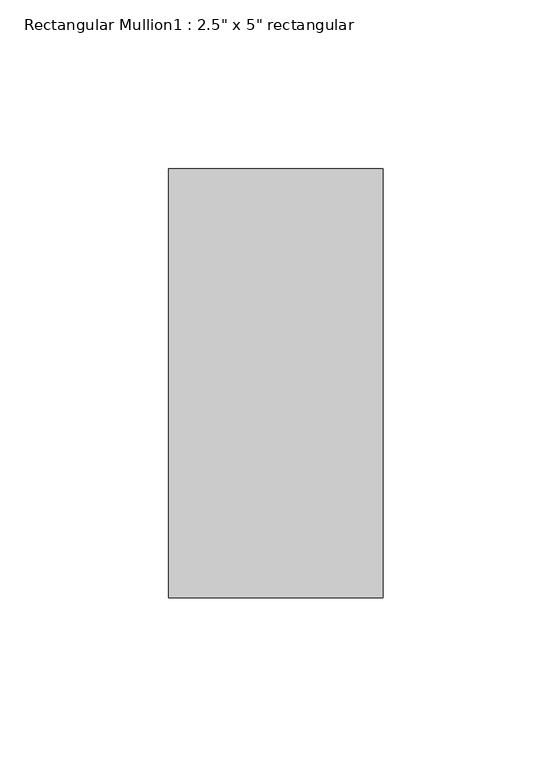
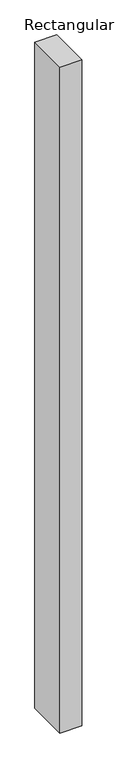
"""IFC4 building model written with IfcOpenShell, lengths in millimetres: member geometry."""

from ifc_helpers import new_model, si_unit, frame, origin, place, context, project, spatial, polyline, outline, extrude, source, transform, mapped, element, save


def member_08becc7e(model_context):
    return source(origin(), model_context, "Body", "SweptSolid", [
        extrude(outline(polyline([(0.0, 63.5), (0.0, -63.5), (-63.5, -63.5), (-63.5, 63.5), (0.0, 63.5)])), frame((0.0, 0.0, -2059.94), z_axis=(0.0, 0.0, 1.0), x_axis=(1.0, 0.0, 0.0)), (0.0, 0.0, 1.0), 2059.94),
    ])


if __name__ == "__main__":
    model = new_model("IFC4")
    model_context = context("Model", 3, world=origin())
    ifc_project = project(units=[si_unit("LENGTHUNIT", "METRE", prefix="MILLI")], contexts=[model_context])
    site = spatial("IfcSite", under=ifc_project)
    building = spatial("IfcBuilding", under=site)
    placement = place(None, origin())
    member_shape = member_08becc7e(model_context)
    element("IfcMember", 1, ObjectType="Rectangular Mullion1 : 2.5\" x 5\" rectangular", at=placement, inside=building, context=model_context, shape_type="MappedRepresentation", body=[
        mapped(member_shape, transform((0.0, 0.0, 0.0), x_axis=(1.0, 0.0, 0.0), y_axis=(0.0, 1.0, 0.0), z_axis=(0.0, 0.0, 1.0))),
    ])
    save(model, "model.ifc")

# Revit data of these elements
# Type "Rectangular Mullion1 : 2.5\" x 5\" rectangular"
#   built-in parameter 1007304 = 0.416667 (stored number, unit not read)
#   built-in parameter 1007301 = 0.104167 (stored number, unit not read)
#   built-in parameter 1007300 = 0.104167 (stored number, unit not read)
# Element 1 (IfcMember, "Rectangular Mullion1 : 2.5\" x 5\" rectangular")
#   Materials on its faces: "support-frame"
# Materials
#   "support-frame": class "Unassigned", colour RGB 233 233 233, transparency 0, Cost = 0
